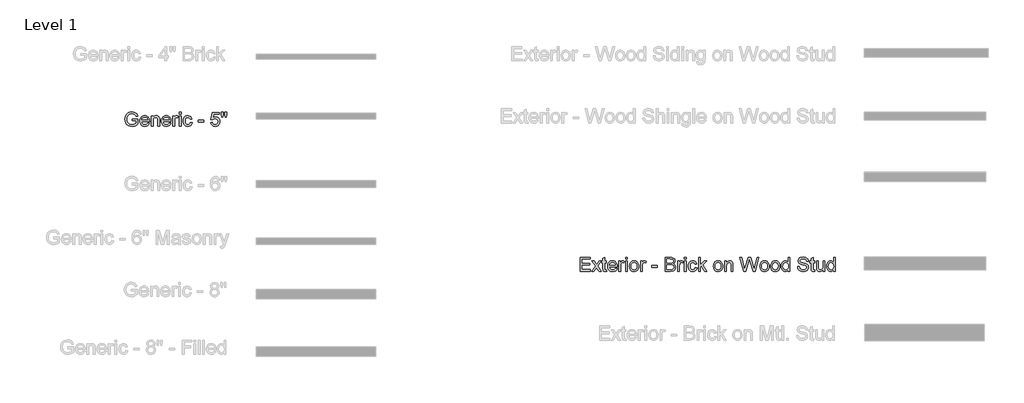
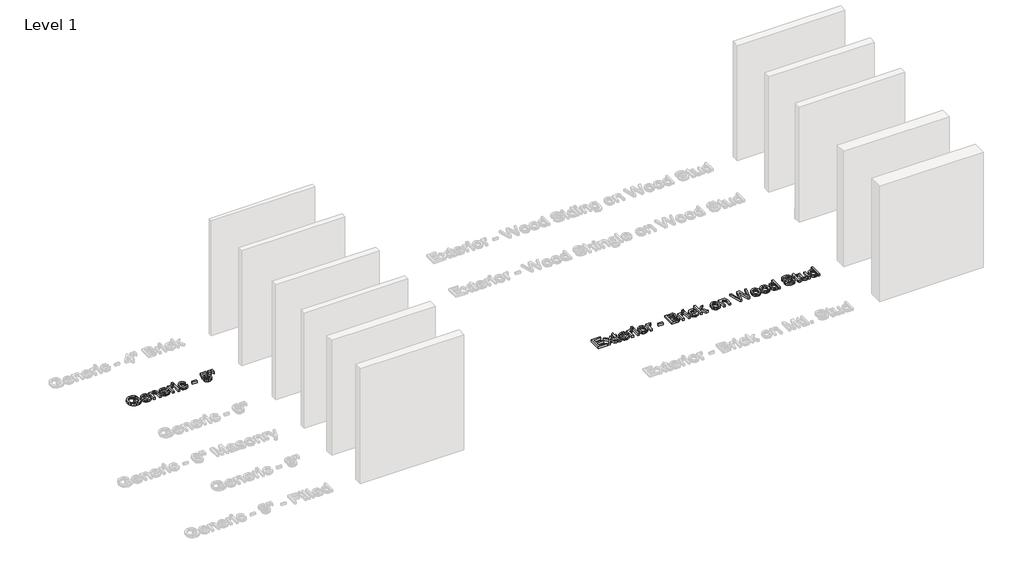
# One storey, part 28 of 42: 2 proxies.
"""IFC4 building model written with IfcOpenShell, lengths in millimetres."""

from ifc_helpers import new_model, si_unit, origin, origin_with_axes, place, context, project, spatial, polyline, outline, extrude, element, save

model = new_model("IFC4")

# Units and contexts
model_context = context("Model", 3, world=origin())
ifc_project = project(units=[si_unit("LENGTHUNIT", "METRE", prefix="MILLI")], contexts=[model_context])

# Site, building, storey
site = spatial("IfcSite", under=ifc_project)
building = spatial("IfcBuilding", under=site)
storey = spatial("IfcBuildingStorey", under=building, Name="Level 1", Elevation=0.0)

# Proxies
placement = place(None, origin())
element("IfcBuildingElementProxy", 1, Name="8\" Arial", ObjectType="8\" Arial", at=placement, inside=storey, context=model_context, shape_type="SweptSolid", body=[
    extrude(outline(polyline([(-15218.2716605, 16003.7864432), (-15218.2716605, 16041.85733), (-15094.5412786, 16041.85733), (-15094.5412786, 15928.0164557), (-15124.6094716, 15907.103493), (-15155.6257189, 15892.1019278), (-15187.5156634, 15883.0675279), (-15220.2049477, 15880.0560613), (-15262.9138649, 15884.8428061), (-15301.5145467, 15899.2030404), (-15333.5810895, 15922.6348533), (-15356.6875896, 15954.6363336), (-15370.6574487, 15993.0232384), (-15375.3140684, 16035.6113251), (-15370.676038, 16078.5061353), (-15356.7619468, 16118.4080681), (-15334.1480632, 16151.8781031), (-15319.7947998, 16164.9115262), (-15303.4106553, 16175.4772196), (-15265.9718048, 16189.4749627), (-15223.253593, 16194.140877), (-15191.8934436, 16191.4361338), (-15163.6934752, 16183.3219043), (-15139.9456442, 16170.3837514), (-15121.941907, 16153.207238), (-15108.6226734, 16130.9651404), (-15098.9283534, 16102.8302346), (-15134.0249521, 16092.9407269), (-15141.8603421, 16113.0078764), (-15151.3873585, 16128.1488614), (-15163.990904, 16139.5626917), (-15181.0558816, 16148.4483772), (-15201.4018706, 16154.164587), (-15223.8484506, 16156.0699903), (-15250.1244264, 16154.0158726), (-15272.5895956, 16147.8535196), (-15291.1603065, 16138.3543872), (-15305.7529071, 16126.2899314), (-15325.3460295, 16096.9560157), (-15334.2688936, 16068.2169576), (-15337.2431816, 16037.1728263), (-15333.6647414, 16000.7656819), (-15322.9294205, 15970.8090247), (-15305.3625318, 15947.5166316), (-15281.2893881, 15931.1022795), (-15253.1173037, 15921.3707809), (-15223.253593, 15918.126948), (-15196.8846707, 15920.571441), (-15171.1663739, 15927.9049199), (-15148.8313297, 15938.0082046), (-15132.6121653, 15948.7621147), (-15132.6121653, 16003.7864432), (-15218.2716605, 16003.7864432)])), origin_with_axes(), (0.0, 0.0, 1.0), 50.8),
    extrude(outline(polyline([(-14880.8386837, 15951.4389739), (-14843.511369, 15946.6801131), (-14856.9607277, 15918.5545019), (-14878.4220747, 15897.5300034), (-14907.4120883, 15884.4245468), (-14943.4474467, 15880.0560613), (-14967.0697999, 15881.9405516), (-14988.117535, 15887.5940225), (-15006.5906521, 15897.016474), (-15022.4891511, 15910.2079061), (-15035.2739423, 15926.8011802), (-15044.405936, 15946.4291575), (-15049.8851322, 15969.0918381), (-15051.7115309, 15994.7892219), (-15049.8665429, 16021.3579792), (-15044.3315788, 16044.7758501), (-15035.1066386, 16065.0428346), (-15022.1917223, 16082.1589328), (-15006.3350492, 16095.7570058), (-14988.2848387, 16105.4699152), (-14968.0410909, 16111.2976608), (-14945.6038055, 16113.2402427), (-14923.8891793, 16111.3023081), (-14904.2519073, 16105.4885045), (-14886.6919896, 16095.7988318), (-14871.2094262, 16082.23329), (-14858.5710258, 16065.1543704), (-14849.5435969, 16044.9245645), (-14844.1271396, 16021.5438722), (-14842.3216538, 15995.0122935), (-14842.5447254, 15984.7509998), (-15013.6406442, 15984.7509998), (-15007.0507373, 15956.2536027), (-14991.7424486, 15935.3034614), (-14969.6490653, 15922.4210764), (-14942.7038747, 15918.126948), (-14922.4415375, 15920.1160031), (-14905.37656, 15926.0831685), (-14891.508942, 15936.4002301), (-14880.8386837, 15951.4389739)]), holes=[polyline([(-15013.6406442, 16022.8218866), (-14880.3925405, 16022.8218866), (-14885.5417767, 16042.9355094), (-14895.6357667, 16057.3236277), (-14917.8313911, 16070.7079239), (-14945.7525199, 16075.1693559), (-14971.4150488, 16071.6095049), (-14992.634735, 16060.929952), (-15007.3853447, 16044.2832337), (-15013.6406442, 16022.8218866)])]), origin_with_axes(), (0.0, 0.0, 1.0), 50.8),
    extrude(outline(polyline([(-14804.250767, 15884.8149221), (-14804.250767, 16108.4813818), (-14766.1798803, 16108.4813818), (-14766.1798803, 16077.2513575), (-14752.9535932, 16092.9964948), (-14737.0690362, 16104.2430214), (-14718.5262093, 16110.9909373), (-14697.3251124, 16113.2402427), (-14678.5592139, 16111.4277859), (-14661.3734059, 16105.9904156), (-14647.0410554, 16097.6066412), (-14636.8355296, 16086.9549722), (-14625.4216993, 16058.9594861), (-14623.4140549, 16022.1526718), (-14623.4140549, 15884.8149221), (-14661.4849417, 15884.8149221), (-14661.4849417, 16017.0220249), (-14665.8720165, 16050.7058369), (-14671.941423, 16060.7347643), (-14681.3754929, 16068.5143864), (-14693.4678326, 16073.5056135), (-14707.5120489, 16075.1693559), (-14729.8099145, 16071.4329066), (-14748.8174739, 16060.2235586), (-14756.4135267, 16051.0729755), (-14761.8392787, 16038.5670238), (-14766.1798803, 16003.4890144), (-14766.1798803, 15884.8149221), (-14804.250767, 15884.8149221)])), origin_with_axes(), (0.0, 0.0, 1.0), 50.8),
    extrude(outline(polyline([(-14414.4703209, 15951.4389739), (-14377.1430062, 15946.6801131), (-14390.5923649, 15918.5545019), (-14412.0537119, 15897.5300034), (-14441.0437255, 15884.4245468), (-14477.0790839, 15880.0560613), (-14500.7014371, 15881.9405516), (-14521.7491723, 15887.5940225), (-14540.2222893, 15897.016474), (-14556.1207883, 15910.2079061), (-14568.9055795, 15926.8011802), (-14578.0375732, 15946.4291575), (-14583.5167694, 15969.0918381), (-14585.3431682, 15994.7892219), (-14583.4981801, 16021.3579792), (-14577.963216, 16044.7758501), (-14568.7382758, 16065.0428346), (-14555.8233595, 16082.1589328), (-14539.9666864, 16095.7570058), (-14521.916476, 16105.4699152), (-14501.6727281, 16111.2976608), (-14479.2354428, 16113.2402427), (-14457.5208165, 16111.3023081), (-14437.8835445, 16105.4885045), (-14420.3236268, 16095.7988318), (-14404.8410635, 16082.23329), (-14392.202663, 16065.1543704), (-14383.1752341, 16044.9245645), (-14377.7587768, 16021.5438722), (-14375.953291, 15995.0122935), (-14376.1763626, 15984.7509998), (-14547.2722814, 15984.7509998), (-14540.6823745, 15956.2536027), (-14525.3740858, 15935.3034614), (-14503.2807025, 15922.4210764), (-14476.3355119, 15918.126948), (-14456.0731747, 15920.1160031), (-14439.0081972, 15926.0831685), (-14425.1405792, 15936.4002301), (-14414.4703209, 15951.4389739)]), holes=[polyline([(-14547.2722814, 16022.8218866), (-14414.0241777, 16022.8218866), (-14419.1734139, 16042.9355094), (-14429.2674039, 16057.3236277), (-14451.4630283, 16070.7079239), (-14479.3841572, 16075.1693559), (-14505.046686, 16071.6095049), (-14526.2663722, 16060.929952), (-14541.0169819, 16044.2832337), (-14547.2722814, 16022.8218866)])]), origin_with_axes(), (0.0, 0.0, 1.0), 50.8),
    extrude(outline(polyline([(-14337.8824042, 15884.8149221), (-14337.8824042, 16108.4813818), (-14304.5703783, 16108.4813818), (-14304.5703783, 16075.3924275), (-14292.2642616, 16094.5765853), (-14280.9247885, 16105.8788798), (-14269.5481368, 16111.3999019), (-14257.1304843, 16113.2402427), (-14238.1693981, 16110.3031332), (-14218.9108831, 16101.4918049), (-14231.6259644, 16067.3618498), (-14245.0102605, 16073.2174794), (-14258.3945567, 16075.1693559), (-14269.7619137, 16073.2918366), (-14279.9209663, 16067.6592786), (-14288.1281423, 16058.6992359), (-14293.6398698, 16046.8392624), (-14298.2686056, 16025.573103), (-14299.8115175, 16002.3736564), (-14299.8115175, 15884.8149221), (-14337.8824042, 15884.8149221)])), origin_with_axes(), (0.0, 0.0, 1.0), 50.8),
    extrude(outline(polyline([(-14195.1165789, 16151.3111294), (-14195.1165789, 16189.3820162), (-14157.0456921, 16189.3820162), (-14157.0456921, 16151.3111294), (-14195.1165789, 16151.3111294)])), origin_with_axes(), (0.0, 0.0, 1.0), 50.8),
    extrude(outline(polyline([(-14195.1165789, 15884.8149221), (-14195.1165789, 16108.4813818), (-14157.0456921, 16108.4813818), (-14157.0456921, 15884.8149221), (-14195.1165789, 15884.8149221)])), origin_with_axes(), (0.0, 0.0, 1.0), 50.8),
    extrude(outline(polyline([(-13957.1735366, 15965.7155565), (-13919.1026499, 15960.9566956), (-13929.7171403, 15927.0962853), (-13949.6634594, 15901.5081137), (-13977.0640878, 15885.4190744), (-14010.0415063, 15880.0560613), (-14031.3936413, 15881.9266096), (-14050.5382968, 15887.5382546), (-14067.4754729, 15896.8909962), (-14082.2051696, 15909.9848345), (-14094.127882, 15926.5734613), (-14102.6441052, 15946.4105682), (-14107.753839, 15969.4961554), (-14109.4570837, 15995.8302227), (-14106.5478582, 16029.7092223), (-14097.8201818, 16059.0710219), (-14083.1346346, 16082.7816743), (-14062.351797, 16099.7072321), (-14037.488608, 16109.85699), (-14010.5620067, 16113.2402427), (-13978.3932228, 16108.5929176), (-13952.674926, 16094.6509425), (-13934.2250456, 16072.1578893), (-13923.8615107, 16041.85733), (-13961.9323975, 16037.0984691), (-13968.8383225, 16053.7080088), (-13979.5922327, 16065.6144556), (-13993.5992703, 16072.7806308), (-14010.2645779, 16075.1693559), (-14034.8675167, 16070.4662629), (-14054.3955766, 16056.3569841), (-14067.1385418, 16032.0793581), (-14071.3861969, 15996.8712236), (-14067.2314883, 15961.1890619), (-14054.7673626, 15936.827784), (-14035.5924994, 15922.802157), (-14011.3055787, 15918.126948), (-13991.5916259, 15921.0454681), (-13975.4282294, 15929.8010285), (-13963.6704971, 15944.6167008), (-13957.1735366, 15965.7155565)])), origin_with_axes(), (0.0, 0.0, 1.0), 50.8),
    extrude(outline(polyline([(-13785.8545462, 15975.2332782), (-13785.8545462, 16013.3041649), (-13666.8830251, 16013.3041649), (-13666.8830251, 15975.2332782), (-13785.8545462, 15975.2332782)])), origin_with_axes(), (0.0, 0.0, 1.0), 50.8),
    extrude(outline(polyline([(-13514.5994781, 15965.7155565), (-13476.5285913, 15970.4744173), (-13469.5390144, 15947.6188727), (-13457.3444335, 15931.2509939), (-13440.0006165, 15921.4079595), (-13417.5633312, 15918.126948), (-13390.2742385, 15922.6906212), (-13369.8260083, 15936.3816408), (-13357.0551591, 15957.6199162), (-13352.7982093, 15984.825357), (-13356.7856142, 16010.4414127), (-13368.7478289, 16030.0345351), (-13388.7777998, 16042.4707769), (-13416.9684736, 16046.6161908), (-13435.4369433, 16044.9617431), (-13450.3920353, 16039.9984), (-13471.7697305, 16022.8218866), (-13509.8406172, 16027.5807474), (-13476.5285913, 16184.6231553), (-13329.0039051, 16184.6231553), (-13329.0039051, 16146.5522686), (-13445.7447102, 16146.5522686), (-13462.0289372, 16062.6773462), (-13434.832791, 16079.1846447), (-13406.3353939, 16084.6870776), (-13387.7948906, 16082.9815093), (-13370.764768, 16077.8648044), (-13355.245026, 16069.336963), (-13341.2356646, 16057.3979849), (-13329.638265, 16042.7775003), (-13321.3544081, 16026.2051392), (-13316.384094, 16007.6809016), (-13314.7273226, 15987.2047875), (-13320.6944879, 15949.1339007), (-13328.1534446, 15932.1618696), (-13338.595984, 15916.5654468), (-13354.4154785, 15900.5925906), (-13372.8746535, 15889.1834076), (-13393.9735092, 15882.3378979), (-13417.7120456, 15880.0560613), (-13437.3586122, 15881.5222923), (-13455.1044229, 15885.9209855), (-13470.9494776, 15893.2521407), (-13484.8937764, 15903.5157581), (-13496.4958234, 15916.2006318), (-13505.3141226, 15930.7955561), (-13511.3486742, 15947.300531), (-13514.5994781, 15965.7155565)])), origin_with_axes(), (0.0, 0.0, 1.0), 50.8),
    extrude(outline(polyline([(-13272.1206466, 16079.9282167), (-13281.4152967, 16138.7447625), (-13281.4152967, 16189.3820162), (-13243.3444099, 16189.3820162), (-13243.3444099, 16138.7447625), (-13251.6724164, 16079.9282167), (-13272.1206466, 16079.9282167)])), origin_with_axes(), (0.0, 0.0, 1.0), 50.8),
    extrude(outline(polyline([(-13196.2019447, 16079.9282167), (-13205.2735232, 16138.7447625), (-13205.2735232, 16189.3820162), (-13167.2026364, 16189.3820162), (-13167.2026364, 16138.7447625), (-13176.1255005, 16079.9282167), (-13196.2019447, 16079.9282167)])), origin_with_axes(), (0.0, 0.0, 1.0), 50.8),
])
element("IfcBuildingElementProxy", 2, Name="8\" Arial", ObjectType="8\" Arial", at=placement, inside=storey, context=model_context, shape_type="SweptSolid", body=[
    extrude(outline(polyline([(-5495.6172996, 12730.6027707), (-5495.6172996, 13035.1698648), (-5276.7097007, 13035.1698648), (-5276.7097007, 12997.0989781), (-5457.5464128, 12997.0989781), (-5457.5464128, 12906.680622), (-5286.2274224, 12906.680622), (-5286.2274224, 12868.6097352), (-5457.5464128, 12868.6097352), (-5457.5464128, 12768.6736575), (-5271.9508399, 12768.6736575), (-5271.9508399, 12730.6027707), (-5495.6172996, 12730.6027707)])), origin_with_axes(), (0.0, 0.0, 1.0), 50.8),
    extrude(outline(polyline([(-5243.3976748, 12730.6027707), (-5162.0508972, 12843.0308582), (-5238.638814, 12954.2692304), (-5192.8347783, 12954.2692304), (-5155.8792496, 12900.7320459), (-5138.628379, 12875.4505977), (-5123.6825817, 12896.1218995), (-5081.5964061, 12954.2692304), (-5035.7923704, 12954.2692304), (-5116.2468616, 12843.0308582), (-5038.7666585, 12730.6027707), (-5084.5706941, 12730.6027707), (-5131.1926589, 12798.1934662), (-5139.743737, 12810.5367615), (-5197.5936392, 12730.6027707), (-5243.3976748, 12730.6027707)])), origin_with_axes(), (0.0, 0.0, 1.0), 50.8),
    extrude(outline(polyline([(-4924.5539982, 12762.3532954), (-4919.7951373, 12729.4874127), (-4948.2739452, 12725.8439099), (-4966.5472273, 12727.4240004), (-4980.1731843, 12732.164272), (-4989.8024418, 12739.4698669), (-4996.0856253, 12748.7459277), (-4999.5432351, 12764.676958), (-5000.6957717, 12791.9474613), (-5000.6957717, 12916.1983437), (-5029.2489368, 12916.1983437), (-5029.2489368, 12954.2692304), (-5000.6957717, 12954.2692304), (-5000.6957717, 13008.6243442), (-4962.624885, 13031.0058616), (-4962.624885, 12954.2692304), (-4924.5539982, 12954.2692304), (-4924.5539982, 12916.1983437), (-4962.624885, 12916.1983437), (-4962.624885, 12793.0628193), (-4960.6172405, 12773.4325183), (-4954.1109855, 12766.4801201), (-4941.135654, 12763.9147967), (-4924.5539982, 12762.3532954)])), origin_with_axes(), (0.0, 0.0, 1.0), 50.8),
    extrude(outline(polyline([(-4729.8868468, 12797.2268226), (-4692.559532, 12792.4679617), (-4706.0088907, 12764.3423506), (-4727.4702377, 12743.3178521), (-4756.4602514, 12730.2123954), (-4792.4956098, 12725.8439099), (-4816.1179629, 12727.7284002), (-4837.1656981, 12733.3818711), (-4855.6388151, 12742.8043226), (-4871.5373141, 12755.9957548), (-4884.3221053, 12772.5890288), (-4893.454099, 12792.2170062), (-4898.9332952, 12814.8796867), (-4900.759694, 12840.5770706), (-4898.9147059, 12867.1458279), (-4893.3797418, 12890.5636987), (-4884.1548016, 12910.8306833), (-4871.2398853, 12927.9467814), (-4855.3832122, 12941.5448545), (-4837.3330018, 12951.2577638), (-4817.0892539, 12957.0855094), (-4794.6519686, 12959.0280913), (-4772.9373423, 12957.0901567), (-4753.3000703, 12951.2763531), (-4735.7401527, 12941.5866804), (-4720.2575893, 12928.0211386), (-4707.6191888, 12910.9422191), (-4698.5917599, 12890.7124131), (-4693.1753026, 12867.3317209), (-4691.3698168, 12840.8001422), (-4691.5928884, 12830.5388485), (-4862.6888072, 12830.5388485), (-4856.0989003, 12802.0414513), (-4840.7906116, 12781.09131), (-4818.6972283, 12768.208925), (-4791.7520377, 12763.9147967), (-4771.4897006, 12765.9038518), (-4754.424723, 12771.8710171), (-4740.5571051, 12782.1880787), (-4729.8868468, 12797.2268226)]), holes=[polyline([(-4862.6888072, 12868.6097352), (-4729.4407036, 12868.6097352), (-4734.5899397, 12888.723358), (-4744.6839297, 12903.1114764), (-4766.8795541, 12916.4957725), (-4794.800683, 12920.9572045), (-4820.4632119, 12917.3973536), (-4841.682898, 12906.7178006), (-4856.4335077, 12890.0710823), (-4862.6888072, 12868.6097352)])]), origin_with_axes(), (0.0, 0.0, 1.0), 50.8),
    extrude(outline(polyline([(-4653.29893, 12730.6027707), (-4653.29893, 12954.2692304), (-4619.9869041, 12954.2692304), (-4619.9869041, 12921.1802761), (-4607.6807874, 12940.3644339), (-4596.3413143, 12951.6667284), (-4584.9646626, 12957.1877506), (-4572.5470101, 12959.0280913), (-4553.5859239, 12956.0909819), (-4534.3274089, 12947.2796536), (-4547.0424902, 12913.1496985), (-4560.4267864, 12919.005328), (-4573.8110825, 12920.9572045), (-4585.1784395, 12919.0796852), (-4595.3374921, 12913.4471273), (-4603.5446681, 12904.4870846), (-4609.0563956, 12892.6271111), (-4613.6851314, 12871.3609517), (-4615.2280433, 12848.161505), (-4615.2280433, 12730.6027707), (-4653.29893, 12730.6027707)])), origin_with_axes(), (0.0, 0.0, 1.0), 50.8),
    extrude(outline(polyline([(-4510.5331047, 12997.0989781), (-4510.5331047, 13035.1698648), (-4472.4622179, 13035.1698648), (-4472.4622179, 12997.0989781), (-4510.5331047, 12997.0989781)])), origin_with_axes(), (0.0, 0.0, 1.0), 50.8),
    extrude(outline(polyline([(-4510.5331047, 12730.6027707), (-4510.5331047, 12954.2692304), (-4472.4622179, 12954.2692304), (-4472.4622179, 12730.6027707), (-4510.5331047, 12730.6027707)])), origin_with_axes(), (0.0, 0.0, 1.0), 50.8),
    extrude(outline(polyline([(-4424.8736095, 12842.4360006), (-4422.8148445, 12871.4027776), (-4416.6385495, 12896.3635604), (-4406.3447245, 12917.318349), (-4391.9333696, 12934.2671435), (-4377.4244208, 12945.1000581), (-4361.4097387, 12952.8378543), (-4343.8893233, 12957.4805321), (-4324.8631745, 12959.0280913), (-4303.859589, 12957.143601), (-4284.8682952, 12951.4901301), (-4267.8892932, 12942.0676785), (-4252.9225829, 12928.8762464), (-4240.707089, 12912.3619769), (-4231.9817362, 12892.9710131), (-4226.7465246, 12870.7033552), (-4225.001454, 12845.559003), (-4228.0872778, 12807.097741), (-4237.3447493, 12777.8195932), (-4252.5043236, 12755.8935136), (-4273.2964559, 12739.4884562), (-4297.9923411, 12729.2550465), (-4324.8631745, 12725.8439099), (-4346.1734835, 12727.7214292), (-4365.3413757, 12733.3539872), (-4382.366851, 12742.7415838), (-4397.2499094, 12755.884219), (-4409.3352782, 12772.5588212), (-4417.9676845, 12792.5423189), (-4423.1471282, 12815.834712), (-4424.8736095, 12842.4360006)]), holes=[polyline([(-4386.8027227, 12842.5103578), (-4382.3970586, 12808.0550899), (-4369.1800662, 12783.507919), (-4349.289515, 12768.8130773), (-4324.8631745, 12763.9147967), (-4300.5483699, 12768.8409612), (-4280.6949973, 12783.6194548), (-4267.4780049, 12808.4919385), (-4263.0723408, 12843.700073), (-4267.5058889, 12877.1515187), (-4280.8065331, 12901.3640821), (-4300.6877897, 12916.0589239), (-4324.8631745, 12920.9572045), (-4349.289515, 12916.0775132), (-4369.1800662, 12901.4384394), (-4382.3970586, 12876.9470364), (-4386.8027227, 12842.5103578)])]), origin_with_axes(), (0.0, 0.0, 1.0), 50.8),
    extrude(outline(polyline([(-4182.1717064, 12730.6027707), (-4182.1717064, 12954.2692304), (-4148.8596805, 12954.2692304), (-4148.8596805, 12921.1802761), (-4136.5535638, 12940.3644339), (-4125.2140907, 12951.6667284), (-4113.837439, 12957.1877506), (-4101.4197864, 12959.0280913), (-4082.4587003, 12956.0909819), (-4063.2001853, 12947.2796536), (-4075.9152666, 12913.1496985), (-4089.2995627, 12919.005328), (-4102.6838589, 12920.9572045), (-4114.0512159, 12919.0796852), (-4124.2102685, 12913.4471273), (-4132.4174445, 12904.4870846), (-4137.929172, 12892.6271111), (-4142.5579077, 12871.3609517), (-4144.1008196, 12848.161505), (-4144.1008196, 12730.6027707), (-4182.1717064, 12730.6027707)])), origin_with_axes(), (0.0, 0.0, 1.0), 50.8),
    extrude(outline(polyline([(-3939.4698033, 12821.0211268), (-3939.4698033, 12859.0920136), (-3820.4982822, 12859.0920136), (-3820.4982822, 12821.0211268), (-3939.4698033, 12821.0211268)])), origin_with_axes(), (0.0, 0.0, 1.0), 50.8),
    extrude(outline(polyline([(-3653.9381526, 12730.6027707), (-3653.9381526, 13035.1698648), (-3537.7178479, 13035.1698648), (-3505.7535463, 13032.9298541), (-3480.7974108, 13026.2098221), (-3461.6690209, 13014.8424651), (-3447.1879561, 12998.6604793), (-3438.0699043, 12979.6250359), (-3435.0305538, 12959.6973061), (-3437.5865825, 12941.3589615), (-3445.2546689, 12924.1173856), (-3458.0905806, 12909.0321685), (-3476.1500858, 12897.1629003), (-3454.5772029, 12885.8977844), (-3438.636878, 12868.7584496), (-3428.7938436, 12846.8788433), (-3425.5128321, 12821.3929128), (-3427.7528427, 12800.1546373), (-3434.4728748, 12780.4592738), (-3444.5018022, 12763.7103144), (-3456.6684992, 12751.3112511), (-3471.5678233, 12742.3326192), (-3489.7946321, 12735.8449534), (-3538.6101343, 12730.6027707), (-3653.9381526, 12730.6027707)]), holes=[polyline([(-3615.8672659, 12911.4394828), (-3546.3432832, 12911.4394828), (-3505.7442516, 12914.7111997), (-3491.5327316, 12920.3530523), (-3481.3179112, 12928.8018892), (-3475.1555582, 12939.9275854), (-3473.1014405, 12953.6000156), (-3475.0161384, 12966.872776), (-3480.7602322, 12978.4353207), (-3490.0734716, 12987.4604259), (-3502.6956064, 12993.1208678), (-3551.6226445, 12997.0989781), (-3615.8672659, 12997.0989781), (-3615.8672659, 12911.4394828)]), polyline([(-3615.8672659, 12768.6736575), (-3537.7922051, 12768.6736575), (-3509.5364689, 12770.1608015), (-3485.6306288, 12778.4516294), (-3469.7925451, 12795.3678926), (-3465.1359254, 12807.3208126), (-3463.5837188, 12821.0211268), (-3465.4054703, 12836.9335677), (-3470.8707245, 12850.6152927), (-3480.4163301, 12861.3134349), (-3494.4791357, 12868.2751278), (-3514.3975709, 12872.095229), (-3541.5100652, 12873.3685961), (-3615.8672659, 12873.3685961), (-3615.8672659, 12768.6736575)])]), origin_with_axes(), (0.0, 0.0, 1.0), 50.8),
    extrude(outline(polyline([(-3377.9242236, 12730.6027707), (-3377.9242236, 12954.2692304), (-3344.6121977, 12954.2692304), (-3344.6121977, 12921.1802761), (-3332.306081, 12940.3644339), (-3320.9666079, 12951.6667284), (-3309.5899562, 12957.1877506), (-3297.1723037, 12959.0280913), (-3278.2112175, 12956.0909819), (-3258.9527025, 12947.2796536), (-3271.6677838, 12913.1496985), (-3285.05208, 12919.005328), (-3298.4363761, 12920.9572045), (-3309.8037331, 12919.0796852), (-3319.9627857, 12913.4471273), (-3328.1699617, 12904.4870846), (-3333.6816892, 12892.6271111), (-3338.310425, 12871.3609517), (-3339.8533369, 12848.161505), (-3339.8533369, 12730.6027707), (-3377.9242236, 12730.6027707)])), origin_with_axes(), (0.0, 0.0, 1.0), 50.8),
    extrude(outline(polyline([(-3235.1583983, 12730.6027707), (-3235.1583983, 12954.2692304), (-3197.0875115, 12954.2692304), (-3197.0875115, 12730.6027707), (-3235.1583983, 12730.6027707)])), origin_with_axes(), (0.0, 0.0, 1.0), 50.8),
    extrude(outline(polyline([(-3235.1583983, 12997.0989781), (-3235.1583983, 13035.1698648), (-3197.0875115, 13035.1698648), (-3197.0875115, 12997.0989781), (-3235.1583983, 12997.0989781)])), origin_with_axes(), (0.0, 0.0, 1.0), 50.8),
    extrude(outline(polyline([(-2997.215356, 12811.5034051), (-2959.1444693, 12806.7445443), (-2969.7589597, 12772.884134), (-2989.7052788, 12747.2959623), (-3017.1059072, 12731.206923), (-3050.0833257, 12725.8439099), (-3071.4354607, 12727.7144582), (-3090.5801162, 12733.3261032), (-3107.5172923, 12742.6788449), (-3122.246989, 12755.7726832), (-3134.1697014, 12772.3613099), (-3142.6859246, 12792.1984169), (-3147.7956584, 12815.284004), (-3149.4989031, 12841.6180714), (-3146.5896776, 12875.497071), (-3137.8620012, 12904.8588706), (-3123.176454, 12928.569523), (-3102.3936164, 12945.4950808), (-3077.5304274, 12955.6448387), (-3050.6038261, 12959.0280913), (-3018.4350422, 12954.3807662), (-2992.7167454, 12940.4387911), (-2974.266865, 12917.9457379), (-2963.9033301, 12887.6451786), (-3001.9742169, 12882.8863178), (-3008.8801419, 12899.4958575), (-3019.6340521, 12911.4023042), (-3033.6410897, 12918.5684795), (-3050.3063973, 12920.9572045), (-3074.9093361, 12916.2541116), (-3094.437396, 12902.1448328), (-3107.1803612, 12877.8672067), (-3111.4280163, 12842.6590722), (-3107.2733077, 12806.9769105), (-3094.809182, 12782.6156326), (-3075.6343188, 12768.5900056), (-3051.3473982, 12763.9147967), (-3031.6334453, 12766.8333168), (-3015.4700488, 12775.5888772), (-3003.7123165, 12790.4045494), (-2997.215356, 12811.5034051)])), origin_with_axes(), (0.0, 0.0, 1.0), 50.8),
    extrude(outline(polyline([(-2925.8324434, 12730.6027707), (-2925.8324434, 13035.1698648), (-2887.7615566, 13035.1698648), (-2887.7615566, 12871.5096661), (-2802.3994902, 12954.2692304), (-2749.7545921, 12954.2692304), (-2836.1576593, 12870.4686653), (-2744.9957313, 12730.6027707), (-2789.4613373, 12730.6027707), (-2863.446752, 12843.9975018), (-2887.7615566, 12820.4262692), (-2887.7615566, 12730.6027707), (-2925.8324434, 12730.6027707)])), origin_with_axes(), (0.0, 0.0, 1.0), 50.8),
    extrude(outline(polyline([(-2602.2299059, 12842.4360006), (-2600.1711409, 12871.4027776), (-2593.9948459, 12896.3635604), (-2583.701021, 12917.318349), (-2569.289666, 12934.2671435), (-2554.7807172, 12945.1000581), (-2538.7660351, 12952.8378543), (-2521.2456197, 12957.4805321), (-2502.219471, 12959.0280913), (-2481.2158854, 12957.143601), (-2462.2245917, 12951.4901301), (-2445.2455896, 12942.0676785), (-2430.2788793, 12928.8762464), (-2418.0633854, 12912.3619769), (-2409.3380327, 12892.9710131), (-2404.102821, 12870.7033552), (-2402.3577504, 12845.559003), (-2405.4435743, 12807.097741), (-2414.7010458, 12777.8195932), (-2429.86062, 12755.8935136), (-2450.6527523, 12739.4884562), (-2475.3486376, 12729.2550465), (-2502.219471, 12725.8439099), (-2523.52978, 12727.7214292), (-2542.6976721, 12733.3539872), (-2559.7231474, 12742.7415838), (-2574.6062059, 12755.884219), (-2586.6915746, 12772.5588212), (-2595.3239809, 12792.5423189), (-2600.5034247, 12815.834712), (-2602.2299059, 12842.4360006)]), holes=[polyline([(-2564.1590192, 12842.5103578), (-2559.753355, 12808.0550899), (-2546.5363626, 12783.507919), (-2526.6458114, 12768.8130773), (-2502.219471, 12763.9147967), (-2477.9046664, 12768.8409612), (-2458.0512938, 12783.6194548), (-2444.8343013, 12808.4919385), (-2440.4286372, 12843.700073), (-2444.8621853, 12877.1515187), (-2458.1628296, 12901.3640821), (-2478.0440861, 12916.0589239), (-2502.219471, 12920.9572045), (-2526.6458114, 12916.0775132), (-2546.5363626, 12901.4384394), (-2559.753355, 12876.9470364), (-2564.1590192, 12842.5103578)])]), origin_with_axes(), (0.0, 0.0, 1.0), 50.8),
    extrude(outline(polyline([(-2359.5280028, 12730.6027707), (-2359.5280028, 12954.2692304), (-2321.4571161, 12954.2692304), (-2321.4571161, 12923.0392062), (-2308.230829, 12938.7843434), (-2292.346272, 12950.03087), (-2273.8034451, 12956.778786), (-2252.6023482, 12959.0280913), (-2233.8364497, 12957.2156345), (-2216.6506417, 12951.7782642), (-2202.3182913, 12943.3944898), (-2192.1127655, 12932.7428208), (-2180.6989352, 12904.7473348), (-2178.6912907, 12867.9405204), (-2178.6912907, 12730.6027707), (-2216.7621775, 12730.6027707), (-2216.7621775, 12862.8098736), (-2221.1492523, 12896.4936855), (-2227.2186588, 12906.5226129), (-2236.6527287, 12914.3022351), (-2248.7450684, 12919.2934622), (-2262.7892847, 12920.9572045), (-2285.0871503, 12917.2207552), (-2304.0947097, 12906.0114072), (-2311.6907625, 12896.8608242), (-2317.1165145, 12884.3548725), (-2321.4571161, 12849.2768631), (-2321.4571161, 12730.6027707), (-2359.5280028, 12730.6027707)])), origin_with_axes(), (0.0, 0.0, 1.0), 50.8),
    extrude(outline(polyline([(-1948.1096114, 12730.6027707), (-2031.1666045, 13035.1698648), (-1991.9060026, 13035.1698648), (-1943.7225365, 12835.0002805), (-1928.8510964, 12773.2094467), (-1912.9386554, 12827.8619893), (-1852.5606085, 13035.1698648), (-1795.9747787, 13035.1698648), (-1752.1040303, 12884.8939622), (-1733.3102478, 12829.1260617), (-1719.4612192, 12773.2094467), (-1705.0359223, 12833.2157077), (-1656.406313, 13035.1698648), (-1617.145711, 13035.1698648), (-1700.2770614, 12730.6027707), (-1740.9504502, 12730.6027707), (-1813.9692213, 12965.571525), (-1824.1561578, 12998.3630505), (-1835.6071667, 12958.8793769), (-1902.1568613, 12730.6027707), (-1948.1096114, 12730.6027707)])), origin_with_axes(), (0.0, 0.0, 1.0), 50.8),
    extrude(outline(polyline([(-1593.3514068, 12842.4360006), (-1591.2926418, 12871.4027776), (-1585.1163468, 12896.3635604), (-1574.8225219, 12917.318349), (-1560.4111669, 12934.2671435), (-1545.9022181, 12945.1000581), (-1529.887536, 12952.8378543), (-1512.3671206, 12957.4805321), (-1493.3409719, 12959.0280913), (-1472.3373863, 12957.143601), (-1453.3460926, 12951.4901301), (-1436.3670905, 12942.0676785), (-1421.4003802, 12928.8762464), (-1409.1848863, 12912.3619769), (-1400.4595336, 12892.9710131), (-1395.2243219, 12870.7033552), (-1393.4792513, 12845.559003), (-1396.5650752, 12807.097741), (-1405.8225467, 12777.8195932), (-1420.9821209, 12755.8935136), (-1441.7742532, 12739.4884562), (-1466.4701385, 12729.2550465), (-1493.3409719, 12725.8439099), (-1514.6512809, 12727.7214292), (-1533.819173, 12733.3539872), (-1550.8446483, 12742.7415838), (-1565.7277068, 12755.884219), (-1577.8130755, 12772.5588212), (-1586.4454818, 12792.5423189), (-1591.6249256, 12815.834712), (-1593.3514068, 12842.4360006)]), holes=[polyline([(-1555.2805201, 12842.5103578), (-1550.8748559, 12808.0550899), (-1537.6578635, 12783.507919), (-1517.7673123, 12768.8130773), (-1493.3409719, 12763.9147967), (-1469.0261673, 12768.8409612), (-1449.1727947, 12783.6194548), (-1435.9558022, 12808.4919385), (-1431.5501381, 12843.700073), (-1435.9836862, 12877.1515187), (-1449.2843305, 12901.3640821), (-1469.165587, 12916.0589239), (-1493.3409719, 12920.9572045), (-1517.7673123, 12916.0775132), (-1537.6578635, 12901.4384394), (-1550.8748559, 12876.9470364), (-1555.2805201, 12842.5103578)])]), origin_with_axes(), (0.0, 0.0, 1.0), 50.8),
    extrude(outline(polyline([(-1360.1672254, 12842.4360006), (-1358.1084604, 12871.4027776), (-1351.9321654, 12896.3635604), (-1341.6383405, 12917.318349), (-1327.2269855, 12934.2671435), (-1312.7180367, 12945.1000581), (-1296.7033546, 12952.8378543), (-1279.1829392, 12957.4805321), (-1260.1567905, 12959.0280913), (-1239.1532049, 12957.143601), (-1220.1619112, 12951.4901301), (-1203.1829091, 12942.0676785), (-1188.2161988, 12928.8762464), (-1176.0007049, 12912.3619769), (-1167.2753522, 12892.9710131), (-1162.0401405, 12870.7033552), (-1160.2950699, 12845.559003), (-1163.3808938, 12807.097741), (-1172.6383653, 12777.8195932), (-1187.7979396, 12755.8935136), (-1208.5900718, 12739.4884562), (-1233.2859571, 12729.2550465), (-1260.1567905, 12725.8439099), (-1281.4670995, 12727.7214292), (-1300.6349916, 12733.3539872), (-1317.6604669, 12742.7415838), (-1332.5435254, 12755.884219), (-1344.6288941, 12772.5588212), (-1353.2613004, 12792.5423189), (-1358.4407442, 12815.834712), (-1360.1672254, 12842.4360006)]), holes=[polyline([(-1322.0963387, 12842.5103578), (-1317.6906745, 12808.0550899), (-1304.4736821, 12783.507919), (-1284.5831309, 12768.8130773), (-1260.1567905, 12763.9147967), (-1235.8419859, 12768.8409612), (-1215.9886133, 12783.6194548), (-1202.7716208, 12808.4919385), (-1198.3659567, 12843.700073), (-1202.7995048, 12877.1515187), (-1216.1001491, 12901.3640821), (-1235.9814056, 12916.0589239), (-1260.1567905, 12920.9572045), (-1284.5831309, 12916.0775132), (-1304.4736821, 12901.4384394), (-1317.6906745, 12876.9470364), (-1322.0963387, 12842.5103578)])]), origin_with_axes(), (0.0, 0.0, 1.0), 50.8),
    extrude(outline(polyline([(-979.4583578, 12730.6027707), (-979.4583578, 12766.5172987), (-990.8489515, 12748.7226911), (-1004.6468596, 12736.0122571), (-1020.852082, 12728.3859967), (-1039.4646188, 12725.8439099), (-1064.0768522, 12729.5245913), (-1086.607084, 12740.5666356), (-1105.679706, 12758.1985869), (-1119.91911, 12781.648989), (-1128.7862061, 12809.9697878), (-1131.7419049, 12842.212929), (-1129.0185724, 12874.0564002), (-1120.848575, 12902.8140476), (-1107.2412072, 12926.8500127), (-1088.2057639, 12944.5284372), (-1065.1829156, 12955.4031778), (-1039.6133332, 12959.0280913), (-1020.9868544, 12956.4348839), (-1004.5167345, 12948.6552618), (-990.55617, 12936.7302257), (-979.4583578, 12921.7007765), (-979.4583578, 13035.1698648), (-941.3874711, 13035.1698648), (-941.3874711, 12730.6027707), (-979.4583578, 12730.6027707)]), holes=[polyline([(-1093.6710181, 12842.3616434), (-1089.3768898, 12807.9249648), (-1076.4945048, 12783.4335618), (-1057.7750795, 12768.794488), (-1035.9698304, 12763.9147967), (-1014.1738759, 12768.5714163), (-995.9284778, 12782.5412754), (-983.5758878, 12806.0846241), (-979.4583578, 12839.4617126), (-983.650245, 12875.9525088), (-996.2259066, 12901.2525463), (-1014.9360372, 12916.03104), (-1037.5313316, 12920.9572045), (-1059.5596523, 12916.2262276), (-1077.6098628, 12902.033297), (-1089.6557293, 12877.6534298), (-1093.6710181, 12842.3616434)])]), origin_with_axes(), (0.0, 0.0, 1.0), 50.8),
    extrude(outline(polyline([(-774.8273415, 12835.2977093), (-736.7564548, 12835.2977093), (-732.3879692, 12814.1709697), (-724.4875166, 12797.189644), (-712.1628106, 12783.7124013), (-694.5215648, 12773.0979109), (-672.9579766, 12766.2105752), (-648.8662435, 12763.9147967), (-627.655852, 12765.6528962), (-609.0851412, 12770.8671949), (-594.0371027, 12779.1208442), (-583.3947283, 12789.9769955), (-577.0650716, 12802.4411213), (-574.955186, 12815.5186939), (-576.5352765, 12828.2616592), (-581.2755481, 12839.2758196), (-590.9048056, 12848.6727108), (-607.1518539, 12856.5638687), (-662.5851471, 12871.1007015), (-698.9737021, 12880.7206643), (-722.2568006, 12889.8758946), (-741.2085921, 12902.6839225), (-754.6393615, 12918.2059881), (-762.6420552, 12936.1074842), (-765.3096198, 12956.0538033), (-762.010019, 12978.3516688), (-752.1112167, 12999.1438011), (-735.873463, 13016.7664576), (-713.5570081, 13029.5558962), (-686.7698266, 13037.3355183), (-657.1198928, 13039.9287257), (-624.9975821, 13037.2146878), (-596.8905602, 13029.0725744), (-573.8026494, 13015.6696889), (-556.7376719, 12997.1733353), (-545.9372885, 12974.7360499), (-541.6431601, 12949.5103696), (-579.7140469, 12949.5103696), (-586.7036237, 12972.2264944), (-601.2776351, 12988.6222572), (-624.0495278, 12998.5489435), (-655.6327488, 13001.8578389), (-687.9595418, 12998.5861221), (-710.1365769, 12988.7709716), (-722.963194, 12974.3270853), (-727.2387331, 12957.1691613), (-724.2086771, 12942.539382), (-715.1185094, 12930.772355), (-693.6292783, 12920.2508111), (-652.9558896, 12909.5061956), (-610.9812498, 12899.3006698), (-585.5882657, 12890.396395), (-563.8852578, 12876.584545), (-548.7442728, 12859.5381568), (-539.8492927, 12839.4431233), (-536.8842993, 12816.4853376), (-540.2954359, 12793.0163461), (-550.5288456, 12770.9415521), (-567.1662693, 12751.9432873), (-589.7894476, 12737.7038834), (-616.9948884, 12728.8089033), (-647.3790995, 12725.8439099), (-684.6785303, 12729.0412695), (-715.3787596, 12738.6333484), (-739.8329839, 12754.6573252), (-758.3944002, 12777.1503784), (-770.3101416, 12804.5510068), (-774.8273415, 12835.2977093)])), origin_with_axes(), (0.0, 0.0, 1.0), 50.8),
    extrude(outline(polyline([(-403.6361956, 12762.3532954), (-398.8773348, 12729.4874127), (-427.3561426, 12725.8439099), (-445.6294247, 12727.4240004), (-459.2553817, 12732.164272), (-468.8846392, 12739.4698669), (-475.1678227, 12748.7459277), (-478.6254325, 12764.676958), (-479.7779691, 12791.9474613), (-479.7779691, 12916.1983437), (-508.3311342, 12916.1983437), (-508.3311342, 12954.2692304), (-479.7779691, 12954.2692304), (-479.7779691, 13008.6243442), (-441.7070824, 13031.0058616), (-441.7070824, 12954.2692304), (-403.6361956, 12954.2692304), (-403.6361956, 12916.1983437), (-441.7070824, 12916.1983437), (-441.7070824, 12793.0628193), (-439.699438, 12773.4325183), (-433.1931829, 12766.4801201), (-420.2178514, 12763.9147967), (-403.6361956, 12762.3532954)])), origin_with_axes(), (0.0, 0.0, 1.0), 50.8),
    extrude(outline(polyline([(-222.7994835, 12730.6027707), (-222.7994835, 12769.0454435), (-236.5741549, 12750.1447726), (-252.616721, 12736.6442933), (-270.9271817, 12728.5440057), (-291.505537, 12725.8439099), (-310.0483639, 12727.7400185), (-327.3085291, 12733.4283444), (-341.7895939, 12741.9794224), (-351.9951197, 12752.4637877), (-358.8638661, 12765.1974584), (-363.3345928, 12780.4964524), (-365.5653089, 12815.8904799), (-365.5653089, 12954.2692304), (-327.4944221, 12954.2692304), (-327.4944221, 12833.8105653), (-325.1893489, 12794.9961065), (-319.6404428, 12782.048659), (-310.1320157, 12772.2056245), (-297.296104, 12765.9875036), (-281.7647437, 12763.9147967), (-265.341097, 12766.0339769), (-249.9770404, 12772.3915175), (-237.3084323, 12782.4018557), (-228.9711312, 12795.4794284), (-224.3423954, 12813.3902191), (-222.7994835, 12837.9002114), (-222.7994835, 12954.2692304), (-184.7285968, 12954.2692304), (-184.7285968, 12730.6027707), (-222.7994835, 12730.6027707)])), origin_with_axes(), (0.0, 0.0, 1.0), 50.8),
    extrude(outline(polyline([(5.625837, 12730.6027707), (5.625837, 12766.5172987), (-5.7647566, 12748.7226911), (-19.5626647, 12736.0122571), (-35.7678871, 12728.3859967), (-54.3804239, 12725.8439099), (-78.9926574, 12729.5245913), (-101.5228892, 12740.5666356), (-120.5955112, 12758.1985869), (-134.8349151, 12781.648989), (-143.7020113, 12809.9697878), (-146.65771, 12842.212929), (-143.9343775, 12874.0564002), (-135.7643801, 12902.8140476), (-122.1570124, 12926.8500127), (-103.121569, 12944.5284372), (-80.0987207, 12955.4031778), (-54.5291383, 12959.0280913), (-35.9026596, 12956.4348839), (-19.4325396, 12948.6552618), (-5.4719752, 12936.7302257), (5.625837, 12921.7007765), (5.625837, 13035.1698648), (43.6967238, 13035.1698648), (43.6967238, 12730.6027707), (5.625837, 12730.6027707)]), holes=[polyline([(-108.5868232, 12842.3616434), (-104.2926949, 12807.9249648), (-91.4103099, 12783.4335618), (-72.6908846, 12768.794488), (-50.8856355, 12763.9147967), (-29.089681, 12768.5714163), (-10.8442829, 12782.5412754), (1.508307, 12806.0846241), (5.625837, 12839.4617126), (1.4339498, 12875.9525088), (-11.1417117, 12901.2525463), (-29.8518423, 12916.03104), (-52.4471367, 12920.9572045), (-74.4754574, 12916.2262276), (-92.5256679, 12902.033297), (-104.5715344, 12877.6534298), (-108.5868232, 12842.3616434)])]), origin_with_axes(), (0.0, 0.0, 1.0), 50.8),
])

save(model, "model.ifc")

# Revit data of these elements
# Elements 1, 2 (IfcBuildingElementProxy, "8\" Arial")
#   Phase Created = New Construction
